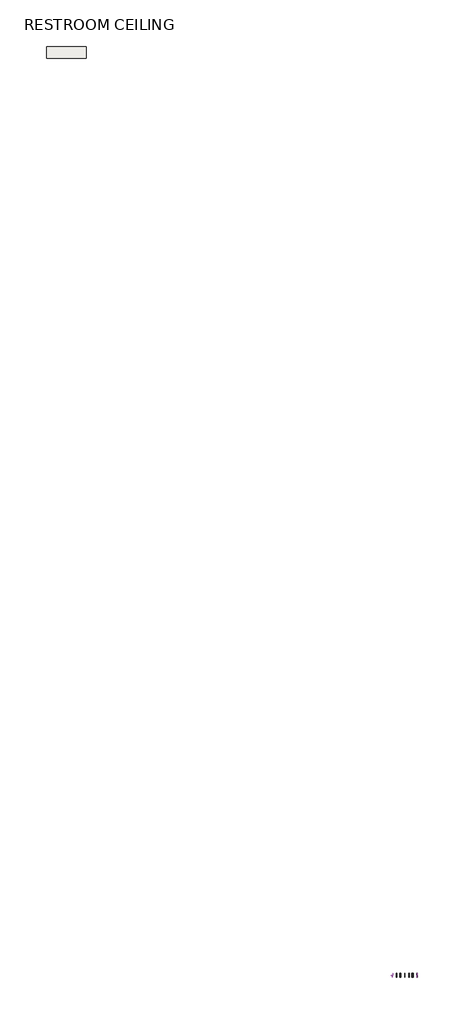
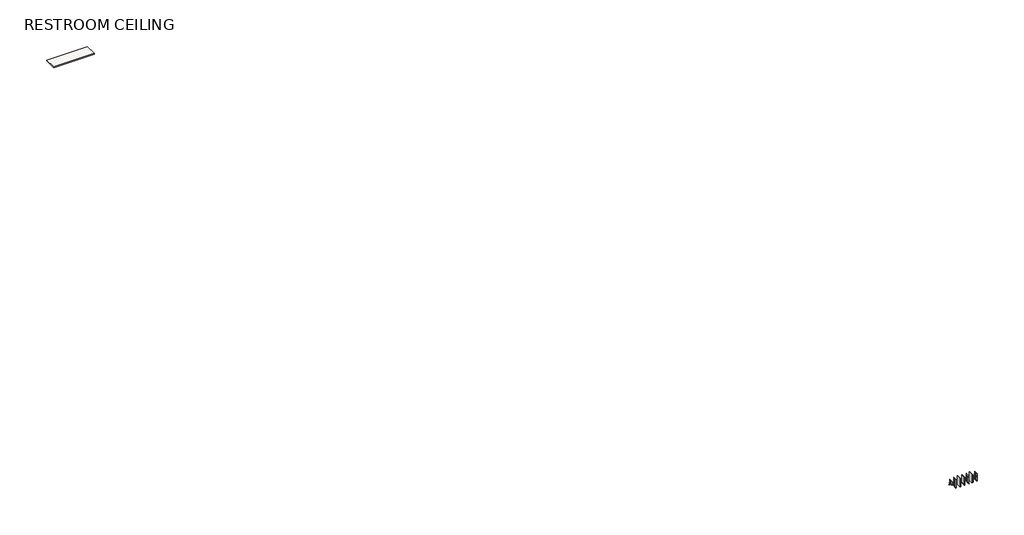
# One storey: 61 proxies, 1 slab.
"""IFC4 building model written with IfcOpenShell, lengths in millimetres."""

import ifcopenshell
import ifcopenshell.guid

model = None  # the IFC model being written
_history = None  # IfcOwnerHistory: only IFC2X3 demands one
_inside = {}  # id of a spatial element -> (the spatial element, [elements in it])
_under = {}  # id of a project, library or spatial element -> (it, [spatial elements below it])
_declared = {}  # id of a project -> (the project, [libraries it declares])
_typed = {}  # id of a type object -> (the type object, [elements of that type])
_made_of = {}  # id of a material, layer set ... -> (it, [elements and type objects made of it])


def new_model(schema):
    """Start an empty IFC model of exactly this schema.

    Asked for "IFC4X3", IfcOpenShell would pick the latest addendum, in which some entities
    have other attributes; the version numbers below select the first issue.
    IFC2X3 requires an IfcOwnerHistory on every rooted entity: one is made here for all.
    """
    global model, _history
    if schema == "IFC4X3":
        model = ifcopenshell.file(schema_version=(4, 3, 0, 0))
    else:
        model = ifcopenshell.file(schema=schema)
    _inside.clear()
    _under.clear()
    _declared.clear()
    _typed.clear()
    _made_of.clear()
    _history = None
    if model.schema == "IFC2X3":
        org = make("IfcOrganization", Name="unknown")
        user = make(
            "IfcPersonAndOrganization",
            ThePerson=make("IfcPerson", FamilyName="unknown"),
            TheOrganization=org,
        )
        app = make(
            "IfcApplication",
            ApplicationDeveloper=org,
            Version="unknown",
            ApplicationFullName="unknown",
            ApplicationIdentifier="unknown",
        )
        _history = make(
            "IfcOwnerHistory",
            OwningUser=user,
            OwningApplication=app,
            ChangeAction="ADDED",
            CreationDate=0,
        )
    return model


def make(cls, **values):
    """One entity of the class cls with the attributes given. An attribute that is None is left unset."""
    return model.create_entity(
        cls, **{name: value for name, value in values.items() if value is not None}
    )


def rooted(cls, **values):
    """An entity with a GlobalId (a new one), such as an element, a storey or a relation."""
    return make(cls, GlobalId=ifcopenshell.guid.new(), OwnerHistory=_history, **values)


def si_unit(unit_type, name, prefix=None):
    """IfcSIUnit, for example si_unit("LENGTHUNIT", "METRE", prefix="MILLI")."""
    return make("IfcSIUnit", UnitType=unit_type, Prefix=prefix, Name=name)


def assignment(units):
    """IfcUnitAssignment: the units of a project."""
    return None if units is None else make("IfcUnitAssignment", Units=units)


def point(xyz):
    """IfcCartesianPoint."""
    return None if xyz is None else make("IfcCartesianPoint", Coordinates=xyz)


def direction(xyz):
    """IfcDirection."""
    return None if xyz is None else make("IfcDirection", DirectionRatios=xyz)


def frame(location, z_axis=None, x_axis=None):
    """IfcAxis2Placement3D, a coordinate frame: its origin and axes. An axis left out is left unset."""
    return make(
        "IfcAxis2Placement3D",
        Location=point(location),
        Axis=direction(z_axis),
        RefDirection=direction(x_axis),
    )


def frame_2d(location, x_axis=None):
    """IfcAxis2Placement2D, a coordinate frame in the plane: its origin and x axis."""
    return make(
        "IfcAxis2Placement2D", Location=point(location), RefDirection=direction(x_axis)
    )


def origin():
    """The frame at (0, 0, 0) with its axes left unset."""
    return frame((0.0, 0.0, 0.0))


def place(relative_to, where):
    """IfcLocalPlacement: puts the frame where relative to a parent placement (None: the world)."""
    return make(
        "IfcLocalPlacement", PlacementRelTo=relative_to, RelativePlacement=where
    )


def context(
    kind, dimensions, precision=None, world=None, true_north=None, identifier=None
):
    """IfcGeometricRepresentationContext, for example the 3D "Model" context."""
    return make(
        "IfcGeometricRepresentationContext",
        ContextIdentifier=identifier,
        ContextType=kind,
        CoordinateSpaceDimension=dimensions,
        Precision=precision,
        WorldCoordinateSystem=world,
        TrueNorth=true_north,
    )


def project(units=None, contexts=None):
    """IfcProject with its units and contexts."""
    return rooted(
        "IfcProject",
        Name="project",
        RepresentationContexts=contexts,
        UnitsInContext=assignment(units),
    )


def spatial(cls, under=None, at=None, **own):
    """A site, building, storey or space (cls), placed at a placement, below another one or the project."""
    s = rooted(cls, ObjectPlacement=at, **own)
    if under is not None:
        _under.setdefault(under.id(), (under, []))[1].append(s)
    return s


def polyline(points):
    """IfcPolyline through the points."""
    return make("IfcPolyline", Points=[point(p) for p in points])


def circle_curve(where, radius):
    """IfcCircle in the frame where."""
    return make("IfcCircle", Position=where, Radius=radius)


def trimmed(basis, trim1, trim2, sense, master):
    """IfcTrimmedCurve: the piece of a basis curve between two trims."""
    return make(
        "IfcTrimmedCurve",
        BasisCurve=basis,
        Trim1=trim1,
        Trim2=trim2,
        SenseAgreement=sense,
        MasterRepresentation=master,
    )


def segment(curve, same_sense, transition):
    """IfcCompositeCurveSegment."""
    return make(
        "IfcCompositeCurveSegment",
        Transition=transition,
        SameSense=same_sense,
        ParentCurve=curve,
    )


def composite_curve(segments, self_intersect=None):
    """IfcCompositeCurve: segments joined end to end."""
    return make("IfcCompositeCurve", Segments=segments, SelfIntersect=self_intersect)


def outline(outer, holes=None, kind="AREA"):
    """IfcArbitraryClosedProfileDef: a profile drawn as a closed curve; with holes, ...WithVoids."""
    if holes is None:
        return make("IfcArbitraryClosedProfileDef", ProfileType=kind, OuterCurve=outer)
    return make(
        "IfcArbitraryProfileDefWithVoids",
        ProfileType=kind,
        OuterCurve=outer,
        InnerCurves=holes,
    )


def extrude(swept, where, along, depth):
    """IfcExtrudedAreaSolid: the profile swept, set in the frame where, extruded along a direction by depth."""
    return make(
        "IfcExtrudedAreaSolid",
        SweptArea=swept,
        Position=where,
        ExtrudedDirection=direction(along),
        Depth=depth,
    )


def shape(context_of_items, identifier, shape_type, items):
    """IfcShapeRepresentation: the items that make up one representation, for example the "Body"."""
    return make(
        "IfcShapeRepresentation",
        ContextOfItems=context_of_items,
        RepresentationIdentifier=identifier,
        RepresentationType=shape_type,
        Items=items,
    )


def source(mapping_origin, context_of_items, identifier, shape_type, items):
    """IfcRepresentationMap: a shape defined once, which mapped items show again and again."""
    return make(
        "IfcRepresentationMap",
        MappingOrigin=mapping_origin,
        MappedRepresentation=shape(context_of_items, identifier, shape_type, items),
    )


def transform(
    local_origin,
    x_axis=None,
    y_axis=None,
    z_axis=None,
    scale=None,
    scale2=None,
    scale3=None,
    uniform=True,
):
    """IfcCartesianTransformationOperator3D, or its non-uniform kind. x_axis, y_axis, z_axis: its Axis1, 2, 3."""
    if uniform:
        return make(
            "IfcCartesianTransformationOperator3D",
            Axis1=direction(x_axis),
            Axis2=direction(y_axis),
            LocalOrigin=point(local_origin),
            Scale=scale,
            Axis3=direction(z_axis),
        )
    return make(
        "IfcCartesianTransformationOperator3DnonUniform",
        Axis1=direction(x_axis),
        Axis2=direction(y_axis),
        LocalOrigin=point(local_origin),
        Scale=scale,
        Axis3=direction(z_axis),
        Scale2=scale2,
        Scale3=scale3,
    )


def mapped(mapping_source, mapping_target):
    """IfcMappedItem: shows the shape of a source again, moved by a transform."""
    return make(
        "IfcMappedItem", MappingSource=mapping_source, MappingTarget=mapping_target
    )


def made_of(thing, what):
    """Note that an element or type object is made of a material, layer set ...; save() writes the relation."""
    if what is not None:
        _made_of.setdefault(what.id(), (what, []))[1].append(thing)
    return thing


def element(
    cls,
    number,
    at=None,
    inside=None,
    cuts=None,
    type_object=None,
    material=None,
    context=None,
    identifier="Body",
    shape_type=None,
    held_by="IfcProductDefinitionShape",
    body=None,
    shapes=None,
    **own,
):
    """One element of the class cls, such as IfcWall. Its Tag is "e" and its number.

    at: its placement. inside: the storey or other place that contains it. cuts: it is an
    opening in that element (IfcRelVoidsElement). A single representation is given by context,
    identifier, shape_type and body (its items); several are given by shapes. held_by: the class
    of the entity that holds the representations. save() writes the other relations.
    """
    e = rooted(cls, Tag="e%d" % number, ObjectPlacement=at, **own)
    if body is not None:
        shapes = [shape(context, identifier, shape_type, body)]
    if shapes is not None:
        e.Representation = make(held_by, Representations=shapes)
    if inside is not None:
        _inside.setdefault(inside.id(), (inside, []))[1].append(e)
    if cuts is not None:
        rooted(
            "IfcRelVoidsElement", RelatingBuildingElement=cuts, RelatedOpeningElement=e
        )
    if type_object is not None:
        _typed.setdefault(type_object.id(), (type_object, []))[1].append(e)
    return made_of(e, material)


def aggregate(whole, parts):
    """IfcRelAggregates: a whole, such as a stair, and the parts it consists of."""
    return rooted("IfcRelAggregates", RelatingObject=whole, RelatedObjects=parts)


def save(model, path):
    """Write the relations noted so far, then the file.

    IfcRelAggregates (storeys below a building ...), IfcRelContainedInSpatialStructure (elements
    in a storey), IfcRelDefinesByType, IfcRelAssociatesMaterial and IfcRelDeclares: one each for
    every whole, place, type object, material and project.
    """
    for whole, parts in _under.values():
        aggregate(whole, parts)
    for where, things in _inside.values():
        rooted(
            "IfcRelContainedInSpatialStructure",
            RelatedElements=things,
            RelatingStructure=where,
        )
    for kind, things in _typed.values():
        rooted("IfcRelDefinesByType", RelatedObjects=things, RelatingType=kind)
    for what, things in _made_of.values():
        rooted("IfcRelAssociatesMaterial", RelatedObjects=things, RelatingMaterial=what)
    for by, libraries in _declared.values():
        rooted("IfcRelDeclares", RelatingContext=by, RelatedDefinitions=libraries)
    model.write(path)


def generic_models_1_generic_models_1_05f3df34(model_context):
    return source(origin(), model_context, "Body", "SweptSolid", [
        extrude(outline(polyline([(49784.0, 0.0), (49695.1, 0.0), (49695.1, 1219.2), (49784.0, 1219.2), (49784.0, 0.0)])), frame((0.0, 0.0, 3048.0), z_axis=(0.0, 0.0, 1.0), x_axis=(1.0, 0.0, 0.0)), (0.0, 0.0, 1.0), 38.1),
    ])


def generic_models_100_generic_models_1_fed90478(model_context):
    return source(origin(), model_context, "Body", "SweptSolid", [
        extrude(outline(polyline([(52216.05, 1219.2), (52216.05, 0.0), (52139.85, 0.0), (52139.85, 1219.2), (52216.05, 1219.2)])), frame((0.0, 0.0, 3211.5125), z_axis=(0.0, 0.0, 1.0), x_axis=(1.0, 0.0, 0.0)), (0.0, 0.0, 1.0), 1155.7),
    ])


def generic_models_101_generic_models_65_cc6b61b5(model_context):
    return source(origin(), model_context, "Body", "SweptSolid", [
        extrude(outline(polyline([(52222.4, 592.1375), (52133.5, 592.1375), (52133.5, 630.2375), (52222.4, 630.2375), (52222.4, 592.1375)])), frame((0.0, 0.0, 3203.178125), z_axis=(0.0, 0.0, 1.0), x_axis=(1.0, 0.0, 0.0)), (0.0, 0.0, 1.0), 1943.1),
    ])


def generic_models_102_generic_models_1_8a2dd616(model_context):
    return source(origin(), model_context, "Body", "SweptSolid", [
        extrude(outline(composite_curve([segment(polyline([(4498.578125, 52222.4), (4510.823229, 52207.8068534), (4508.6950617, 52206.021109), (4497.282664, 52219.621875), (4414.3677682, 52219.621875)]), True, "CONTINUOUS"), segment(trimmed(circle_curve(frame_2d((4414.4412941, 52217.6381931)), 1.9850441), [point((4414.3677682, 52219.621875))], [point((4412.45625, 52217.6381931))], True, "CARTESIAN"), True, "CONTINUOUS"), segment(polyline([(4412.45625, 52217.6381931), (4412.45625, 52023.9610661)]), True, "CONTINUOUS"), segment(trimmed(circle_curve(frame_2d((4414.4419899, 52023.9610661)), 1.9857399), [point((4412.45625, 52023.9610661))], [point((4414.3365981, 52021.978125))], True, "CARTESIAN"), True, "CONTINUOUS"), segment(polyline([(4414.3365981, 52021.978125), (4497.282664, 52021.978125), (4508.718285, 52035.6065673), (4510.8464522, 52033.820823), (4498.578125, 52019.2), (4414.440625, 52019.2)]), True, "CONTINUOUS"), segment(trimmed(circle_curve(frame_2d((4414.440625, 52023.9625)), 4.7625), [point((4414.440625, 52019.2))], [point((4409.678125, 52023.9625))], False, "CARTESIAN"), True, "CONTINUOUS"), segment(polyline([(4409.678125, 52023.9625), (4409.678125, 52217.6375)]), True, "CONTINUOUS"), segment(trimmed(circle_curve(frame_2d((4414.440625, 52217.6375)), 4.7625), [point((4409.678125, 52217.6375))], [point((4414.440625, 52222.4))], False, "CARTESIAN"), True, "CONTINUOUS"), segment(polyline([(4414.440625, 52222.4), (4498.578125, 52222.4)]), True, "CONTINUOUS")], self_intersect=False)), frame((0.0, 0.0, 0.0), z_axis=(0.0, 1.0, 0.0), x_axis=(0.0, 0.0, 1.0)), (0.0, 0.0, 1.0), 1219.2),
    ])


def generic_models_103_generic_models_1_250a6a11(model_context):
    return source(origin(), model_context, "Body", "SweptSolid", [
        extrude(outline(polyline([(49784.0, 0.0), (49695.1, 0.0), (49695.1, 1219.2), (49784.0, 1219.2), (49784.0, 0.0)])), frame((0.0, 0.0, 5264.15), z_axis=(0.0, 0.0, 1.0), x_axis=(1.0, 0.0, 0.0)), (0.0, 0.0, 1.0), 38.1),
    ])


def generic_models_104_generic_models_1_af33e5d9(model_context):
    return source(origin(), model_context, "Body", "SweptSolid", [
        extrude(outline(polyline([(52206.021109, 0.0), (52117.121109, 0.0), (52117.121109, 1219.2), (52206.021109, 1219.2), (52206.021109, 0.0)])), frame((0.0, 0.0, 4412.45625), z_axis=(0.0, 0.0, 1.0), x_axis=(1.0, 0.0, 0.0)), (0.0, 0.0, 1.0), 38.1),
    ])


def generic_models_108_generic_models_1_496acf5e(model_context):
    return source(origin(), model_context, "Body", "SweptSolid", [
        extrude(outline(polyline([(52216.05, 1219.2), (52216.05, 0.0), (52139.85, 0.0), (52139.85, 1219.2), (52216.05, 1219.2)])), frame((0.0, 0.0, 4570.4125), z_axis=(0.0, 0.0, 1.0), x_axis=(1.0, 0.0, 0.0)), (0.0, 0.0, 1.0), 565.15),
    ])


def generic_models_157_generic_models_1_b3b9a6c0(model_context):
    return source(origin(), model_context, "Body", "SweptSolid", [
        extrude(outline(polyline([(47363.0625, 1219.2), (47363.0625, 0.0), (47347.1875, 0.0), (47347.1875, 1219.2), (47363.0625, 1219.2)])), frame((0.0, 0.0, 4267.2), z_axis=(0.0, 0.0, 1.0), x_axis=(1.0, 0.0, 0.0)), (0.0, 0.0, 1.0), 1123.95),
    ])


def generic_models_2_generic_models_1_35b0c06a(model_context):
    return source(origin(), model_context, "Body", "SweptSolid", [
        extrude(outline(polyline([(49799.875, 1219.2), (49799.875, 0.0), (49784.0, 0.0), (49784.0, 1219.2), (49799.875, 1219.2)])), frame((0.0, 0.0, 3054.35), z_axis=(0.0, 0.0, 1.0), x_axis=(1.0, 0.0, 0.0)), (0.0, 0.0, 1.0), 2438.4),
    ])


def generic_models_216_generic_models_1_bf22bbd9(model_context):
    return source(origin(), model_context, "Body", "SweptSolid", [
        extrude(outline(polyline([(48582.2625, 1219.2), (48582.2625, 0.0), (48566.3875, 0.0), (48566.3875, 1219.2), (48582.2625, 1219.2)])), frame((0.0, 0.0, 3054.35), z_axis=(0.0, 0.0, 1.0), x_axis=(1.0, 0.0, 0.0)), (0.0, 0.0, 1.0), 2336.8),
    ])


def generic_models_17_generic_models_1_5a74d62d(model_context):
    return source(origin(), model_context, "Body", "SweptSolid", [
        extrude(outline(composite_curve([segment(trimmed(circle_curve(frame_2d((3.175, 49802.7897405)), 4.3100275), [point((0.0, 49799.875))], [point((6.35, 49799.875))], True, "CARTESIAN"), True, "CONTINUOUS"), segment(polyline([(6.35, 49799.875), (6.35, 49790.35)]), True, "CONTINUOUS"), segment(trimmed(circle_curve(frame_2d((3.175, 49793.2647405)), 4.3100275), [point((6.35, 49790.35))], [point((0.0, 49790.35))], False, "CARTESIAN"), True, "CONTINUOUS"), segment(polyline([(0.0, 49790.35), (0.0, 49799.875)]), True, "CONTINUOUS")], self_intersect=False)), frame((0.0, 0.0, 0.0), z_axis=(0.0, 1.0, 0.0), x_axis=(0.0, 0.0, 1.0)), (0.0, 0.0, 1.0), 1219.2),
    ])


def generic_models_186_generic_models_1_ef70466a(model_context):
    return source(origin(), model_context, "Body", "SweptSolid", [
        extrude(outline(composite_curve([segment(polyline([(101.6, 49799.875), (15.4496307, 49799.875)]), True, "CONTINUOUS"), segment(trimmed(circle_curve(frame_2d((15.4496307, 49817.7146968)), 17.8396968), [point((15.4496307, 49799.875))], [point((0.0, 49808.7948484))], False, "CARTESIAN"), True, "CONTINUOUS"), segment(polyline([(0.0, 49808.7948484), (2.7496307, 49810.3823484)]), True, "CONTINUOUS"), segment(trimmed(circle_curve(frame_2d((15.4496307, 49817.7146968)), 14.6646968), [point((2.7496307, 49810.3823484))], [point((15.4496307, 49803.05))], True, "CARTESIAN"), True, "CONTINUOUS"), segment(polyline([(15.4496307, 49803.05), (99.5131982, 49803.05)]), True, "CONTINUOUS"), segment(trimmed(circle_curve(frame_2d((99.5131982, 49800.9631982)), 2.0868018), [point((99.5131982, 49803.05))], [point((101.6, 49800.9631982))], False, "CARTESIAN"), True, "CONTINUOUS"), segment(polyline([(101.6, 49800.9631982), (101.6, 49799.875)]), True, "CONTINUOUS")], self_intersect=False)), frame((0.0, 0.0, 0.0), z_axis=(0.0, 1.0, 0.0), x_axis=(0.0, 0.0, 1.0)), (0.0, 0.0, 1.0), 1219.2),
    ])


def generic_models_227_generic_models_46_e0d4e21f(model_context):
    return source(origin(), model_context, "Body", "SweptSolid", [
        extrude(outline(polyline([(48566.0211605, 0.0), (48565.2274105, 0.0), (48565.2274105, 1219.2), (48566.0211605, 1219.2), (48566.0211605, 0.0)])), frame((0.0, 0.0, 3049.1358009), z_axis=(0.0, 0.0, 1.0), x_axis=(1.0, 0.0, 0.0)), (0.0, 0.0, 1.0), 2456.7781344),
    ])


def generic_models_228_generic_models_1_053e8907(model_context):
    return source(origin(), model_context, "Body", "SweptSolid", [
        extrude(outline(composite_curve([segment(polyline([(592.1375, 4235.45), (592.1375, 4267.2)]), True, "CONTINUOUS"), segment(trimmed(circle_curve(frame_2d((592.1375, 4264.025)), 3.175), [point((592.1375, 4267.2))], [point((595.3125, 4264.025))], False, "CARTESIAN"), True, "CONTINUOUS"), segment(polyline([(595.3125, 4264.025), (595.3125, 4240.2125)]), True, "CONTINUOUS"), segment(trimmed(circle_curve(frame_2d((596.9, 4240.2125)), 1.5875), [point((595.3125, 4240.2125))], [point((596.9, 4238.625))], True, "CARTESIAN"), True, "CONTINUOUS"), segment(polyline([(596.9, 4238.625), (620.7125, 4238.625)]), True, "CONTINUOUS"), segment(trimmed(circle_curve(frame_2d((620.7125, 4235.45)), 3.175), [point((620.7125, 4238.625))], [point((623.8875, 4235.45))], False, "CARTESIAN"), True, "CONTINUOUS"), segment(polyline([(623.8875, 4235.45), (592.1375, 4235.45)]), True, "CONTINUOUS")], self_intersect=False)), frame((46753.4625, 0.0, 0.0), z_axis=(1.0, 0.0, 0.0), x_axis=(0.0, 1.0, 0.0)), (0.0, 0.0, 1.0), 609.6),
    ])


def generic_models_232_generic_models_1_b4b06e59(model_context):
    return source(origin(), model_context, "Body", "SweptSolid", [
        extrude(outline(polyline([(49777.65, 1219.2), (49777.65, 0.0), (49701.45, 0.0), (49701.45, 1219.2), (49777.65, 1219.2)])), frame((0.0, 0.0, 3090.8625), z_axis=(0.0, 0.0, 1.0), x_axis=(1.0, 0.0, 0.0)), (0.0, 0.0, 1.0), 2368.55),
    ])


def generic_models_234_generic_models_65_886ed74c(model_context):
    return source(origin(), model_context, "Body", "SweptSolid", [
        extrude(outline(polyline([(49784.0, 592.1375), (49695.1, 592.1375), (49695.1, 630.2375), (49784.0, 630.2375), (49784.0, 592.1375)])), frame((0.0, 0.0, 3086.1), z_axis=(0.0, 0.0, 1.0), x_axis=(1.0, 0.0, 0.0)), (0.0, 0.0, 1.0), 2381.25),
    ])


def generic_models_241_generic_models_1_d4f8735c(model_context):
    return source(origin(), model_context, "Body", "SweptSolid", [
        extrude(outline(polyline([(48469.55, 1219.2), (48469.55, 0.0), (48317.15, 0.0), (48317.15, 1219.2), (48469.55, 1219.2)])), frame((0.0, 0.0, 3048.0), z_axis=(0.0, 0.0, 1.0), x_axis=(1.0, 0.0, 0.0)), (0.0, 0.0, 1.0), 2633.9569015),
    ])


def generic_models_246_generic_models_1_33f707d8(model_context):
    return source(origin(), model_context, "Body", "SweptSolid", [
        extrude(outline(composite_curve([segment(polyline([(4267.2, 47363.0625), (4267.2, 47331.3125)]), True, "CONTINUOUS"), segment(trimmed(circle_curve(frame_2d((4267.2, 47334.4875)), 3.175), [point((4267.2, 47331.3125))], [point((4264.025, 47334.4875))], False, "CARTESIAN"), True, "CONTINUOUS"), segment(polyline([(4264.025, 47334.4875), (4264.025, 47358.3)]), True, "CONTINUOUS"), segment(trimmed(circle_curve(frame_2d((4262.4375, 47358.3)), 1.5875), [point((4264.025, 47358.3))], [point((4262.4375, 47359.8875))], True, "CARTESIAN"), True, "CONTINUOUS"), segment(polyline([(4262.4375, 47359.8875), (4238.625, 47359.8875)]), True, "CONTINUOUS"), segment(trimmed(circle_curve(frame_2d((4238.625, 47363.0625)), 3.175), [point((4238.625, 47359.8875))], [point((4235.45, 47363.0625))], False, "CARTESIAN"), True, "CONTINUOUS"), segment(polyline([(4235.45, 47363.0625), (4267.2, 47363.0625)]), True, "CONTINUOUS")], self_intersect=False)), frame((0.0, 0.0, 0.0), z_axis=(0.0, 1.0, 0.0), x_axis=(0.0, 0.0, 1.0)), (0.0, 0.0, 1.0), 1219.2),
    ])


def generic_models_248_generic_models_65_f6c484d7(model_context):
    return source(origin(), model_context, "Body", "SweptSolid", [
        extrude(outline(polyline([(47345.6, 592.1375), (47256.7, 592.1375), (47256.7, 630.2375), (47345.6, 630.2375), (47345.6, 592.1375)])), frame((0.0, 0.0, 4305.3), z_axis=(0.0, 0.0, 1.0), x_axis=(1.0, 0.0, 0.0)), (0.0, 0.0, 1.0), 1162.05),
    ])


def generic_models_195_generic_models_1_9bd07d6e(model_context):
    return source(origin(), model_context, "Body", "SweptSolid", [
        extrude(outline(composite_curve([segment(polyline([(0.0, 49676.05), (0.0, 49685.575)]), True, "CONTINUOUS"), segment(trimmed(circle_curve(frame_2d((3.175, 49682.6602595)), 4.3100275), [point((0.0, 49685.575))], [point((6.35, 49685.575))], False, "CARTESIAN"), True, "CONTINUOUS"), segment(polyline([(6.35, 49685.575), (6.35, 49676.05)]), True, "CONTINUOUS"), segment(trimmed(circle_curve(frame_2d((3.175, 49673.1352595)), 4.3100275), [point((6.35, 49676.05))], [point((0.0, 49676.05))], True, "CARTESIAN"), True, "CONTINUOUS")], self_intersect=False)), frame((0.0, 0.0, 0.0), z_axis=(0.0, 1.0, 0.0), x_axis=(0.0, 0.0, 1.0)), (0.0, 0.0, 1.0), 1219.2),
    ])


def generic_models_196_generic_models_1_c5b7b2a8(model_context):
    return source(origin(), model_context, "Body", "SweptSolid", [
        extrude(outline(composite_curve([segment(polyline([(101.6, 49676.05), (101.6, 49674.9618018)]), True, "CONTINUOUS"), segment(trimmed(circle_curve(frame_2d((99.5131982, 49674.9618018)), 2.0868018), [point((101.6, 49674.9618018))], [point((99.5131982, 49672.875))], False, "CARTESIAN"), True, "CONTINUOUS"), segment(polyline([(99.5131982, 49672.875), (15.4496307, 49672.875)]), True, "CONTINUOUS"), segment(trimmed(circle_curve(frame_2d((15.4496307, 49658.2103032)), 14.6646968), [point((15.4496307, 49672.875))], [point((2.7496307, 49665.5426516))], True, "CARTESIAN"), True, "CONTINUOUS"), segment(polyline([(2.7496307, 49665.5426516), (0.0, 49667.1301516)]), True, "CONTINUOUS"), segment(trimmed(circle_curve(frame_2d((15.4496307, 49658.2103032)), 17.8396968), [point((0.0, 49667.1301516))], [point((15.4496307, 49676.05))], False, "CARTESIAN"), True, "CONTINUOUS"), segment(polyline([(15.4496307, 49676.05), (101.6, 49676.05)]), True, "CONTINUOUS")], self_intersect=False)), frame((0.0, 0.0, 0.0), z_axis=(0.0, 1.0, 0.0), x_axis=(0.0, 0.0, 1.0)), (0.0, 0.0, 1.0), 1219.2),
    ])


def generic_models_44_generic_models_1_ce885a63(model_context):
    return source(origin(), model_context, "Body", "SweptSolid", [
        extrude(outline(polyline([(51019.075, 1219.2), (51019.075, 0.0), (51003.2, 0.0), (51003.2, 1219.2), (51019.075, 1219.2)])), frame((0.0, 0.0, 3054.35), z_axis=(0.0, 0.0, 1.0), x_axis=(1.0, 0.0, 0.0)), (0.0, 0.0, 1.0), 2168.128125),
    ])


def generic_models_55_generic_models_1_42571d6e(model_context):
    return source(origin(), model_context, "Body", "SweptSolid", [
        extrude(outline(polyline([(52238.275, 1219.2), (52238.275, 0.0), (52222.4, 0.0), (52222.4, 1219.2), (52238.275, 1219.2)])), frame((0.0, 0.0, 3054.35), z_axis=(0.0, 0.0, 1.0), x_axis=(1.0, 0.0, 0.0)), (0.0, 0.0, 1.0), 2168.128125),
    ])


def generic_models_63_generic_models_1_f1177d32(model_context):
    return source(origin(), model_context, "Body", "SweptSolid", [
        extrude(outline(polyline([(50996.85, 1219.2), (50996.85, 0.0), (50920.65, 0.0), (50920.65, 1219.2), (50996.85, 1219.2)])), frame((0.0, 0.0, 3090.8625), z_axis=(0.0, 0.0, 1.0), x_axis=(1.0, 0.0, 0.0)), (0.0, 0.0, 1.0), 2044.7),
    ])


def generic_models_65_generic_models_65_eaa428f0(model_context):
    return source(origin(), model_context, "Body", "SweptSolid", [
        extrude(outline(polyline([(51003.2, 592.1375), (50914.3, 592.1375), (50914.3, 630.2375), (51003.2, 630.2375), (51003.2, 592.1375)])), frame((0.0, 0.0, 3086.1), z_axis=(0.0, 0.0, 1.0), x_axis=(1.0, 0.0, 0.0)), (0.0, 0.0, 1.0), 2060.178125),
    ])


def generic_models_69_generic_models_1_75d49a3d(model_context):
    return source(origin(), model_context, "Body", "SweptSolid", [
        extrude(outline(polyline([(50914.3, 1219.2), (50914.3, 0.0), (50898.425, 0.0), (50898.425, 1219.2), (50914.3, 1219.2)])), frame((0.0, 0.0, 3054.35), z_axis=(0.0, 0.0, 1.0), x_axis=(1.0, 0.0, 0.0)), (0.0, 0.0, 1.0), 2472.928125),
    ])


def generic_models_76_generic_models_1_e0c76cb0(model_context):
    return source(origin(), model_context, "Body", "SweptSolid", [
        extrude(outline(polyline([(51930.3, 1219.2), (51930.3, 0.0), (51777.9, 0.0), (51777.9, 1219.2), (51930.3, 1219.2)])), frame((0.0, 0.0, 3048.0), z_axis=(0.0, 0.0, 1.0), x_axis=(1.0, 0.0, 0.0)), (0.0, 0.0, 1.0), 2633.9569015),
    ])


def generic_models_85_generic_models_65_bcc3fffd(model_context):
    return source(origin(), model_context, "Body", "SweptSolid", [
        extrude(outline(polyline([(52222.4, 592.1375), (52133.5, 592.1375), (52133.5, 630.2375), (52222.4, 630.2375), (52222.4, 592.1375)])), frame((0.0, 0.0, 3086.1), z_axis=(0.0, 0.0, 1.0), x_axis=(1.0, 0.0, 0.0)), (0.0, 0.0, 1.0), 2098.278125),
    ])


model = new_model("IFC4")

# Units and contexts
model_context = context("Model", 3, world=origin())
ifc_project = project(units=[si_unit("LENGTHUNIT", "METRE", prefix="MILLI")], contexts=[model_context])

# Site, building, storey
site = spatial("IfcSite", under=ifc_project)
building = spatial("IfcBuilding", under=site)
storey = spatial("IfcBuildingStorey", under=building, Name="RESTROOM CEILING", Elevation=3019.425)

# Proxies
placement = place(None, origin())
generic_models_1_generic_models_1_shape = generic_models_1_generic_models_1_05f3df34(model_context)
element("IfcBuildingElementProxy", 1, Name="Generic Models 1 : Generic Models 1", ObjectType="Generic Models 1 : Generic Models 1", at=placement, inside=storey, context=model_context, shape_type="MappedRepresentation", body=[
    mapped(generic_models_1_generic_models_1_shape, transform((0.0, 0.0, 0.0), x_axis=(1.0, 0.0, 0.0), y_axis=(0.0, 1.0, 0.0), z_axis=(0.0, 0.0, 1.0))),
])
generic_models_100_generic_models_1_shape = generic_models_100_generic_models_1_fed90478(model_context)
element("IfcBuildingElementProxy", 2, Name="Generic Models 100 : Generic Models 1", ObjectType="Generic Models 100 : Generic Models 1", at=placement, inside=storey, context=model_context, shape_type="MappedRepresentation", body=[
    mapped(generic_models_100_generic_models_1_shape, transform((1219.2, 0.0, 0.0), x_axis=(1.0, 0.0, 0.0), y_axis=(0.0, 1.0, 0.0), z_axis=(0.0, 0.0, 1.0))),
])
generic_models_101_generic_models_65_shape = generic_models_101_generic_models_65_cc6b61b5(model_context)
element("IfcBuildingElementProxy", 3, Name="Generic Models 101 : Generic Models 65", ObjectType="Generic Models 101 : Generic Models 65", at=placement, inside=storey, context=model_context, shape_type="MappedRepresentation", body=[
    mapped(generic_models_101_generic_models_65_shape, transform((1219.2, 0.0, 0.0), x_axis=(1.0, 0.0, 0.0), y_axis=(0.0, 1.0, 0.0), z_axis=(0.0, 0.0, 1.0))),
])
generic_models_102_generic_models_1_shape = generic_models_102_generic_models_1_8a2dd616(model_context)
element("IfcBuildingElementProxy", 4, Name="Generic Models 102 : Generic Models 1", ObjectType="Generic Models 102 : Generic Models 1", at=placement, inside=storey, context=model_context, shape_type="MappedRepresentation", body=[
    mapped(generic_models_102_generic_models_1_shape, transform((1219.2, 0.0, 0.0), x_axis=(1.0, 0.0, 0.0), y_axis=(0.0, 1.0, 0.0), z_axis=(0.0, 0.0, 1.0))),
])
generic_models_103_generic_models_1_shape = generic_models_103_generic_models_1_250a6a11(model_context)
element("IfcBuildingElementProxy", 5, Name="Generic Models 103 : Generic Models 1", ObjectType="Generic Models 103 : Generic Models 1", at=placement, inside=storey, context=model_context, shape_type="MappedRepresentation", body=[
    mapped(generic_models_103_generic_models_1_shape, transform((3657.6, 0.0, -892.571875), x_axis=(1.0, 0.0, 0.0), y_axis=(0.0, 1.0, 0.0), z_axis=(0.0, 0.0, 1.0))),
])
generic_models_104_generic_models_1_shape = generic_models_104_generic_models_1_af33e5d9(model_context)
element("IfcBuildingElementProxy", 6, Name="Generic Models 104 : Generic Models 1", ObjectType="Generic Models 104 : Generic Models 1", at=placement, inside=storey, context=model_context, shape_type="MappedRepresentation", body=[
    mapped(generic_models_104_generic_models_1_shape, transform((1219.2, 0.0, 0.0), x_axis=(1.0, 0.0, 0.0), y_axis=(0.0, 1.0, 0.0), z_axis=(0.0, 0.0, 1.0))),
])
element("IfcBuildingElementProxy", 7, Name="Generic Models 105 : Generic Models 1", ObjectType="Generic Models 105 : Generic Models 1", at=placement, inside=storey, context=model_context, shape_type="MappedRepresentation", body=[
    mapped(generic_models_103_generic_models_1_shape, transform((3641.221109, 0.0, -813.59375), x_axis=(1.0, 0.0, 0.0), y_axis=(0.0, 1.0, 0.0), z_axis=(0.0, 0.0, 1.0))),
])
element("IfcBuildingElementProxy", 8, Name="Generic Models 106 : Generic Models 1", ObjectType="Generic Models 106 : Generic Models 1", at=placement, inside=storey, context=model_context, shape_type="MappedRepresentation", body=[
    mapped(generic_models_103_generic_models_1_shape, transform((3641.221109, 0.0, -775.49375), x_axis=(1.0, 0.0, 0.0), y_axis=(0.0, 1.0, 0.0), z_axis=(0.0, 0.0, 1.0))),
])
element("IfcBuildingElementProxy", 9, Name="Generic Models 107 : Generic Models 1", ObjectType="Generic Models 107 : Generic Models 1", at=placement, inside=storey, context=model_context, shape_type="MappedRepresentation", body=[
    mapped(generic_models_103_generic_models_1_shape, transform((3657.6, 0.0, -737.39375), x_axis=(1.0, 0.0, 0.0), y_axis=(0.0, 1.0, 0.0), z_axis=(0.0, 0.0, 1.0))),
])
generic_models_108_generic_models_1_shape = generic_models_108_generic_models_1_496acf5e(model_context)
element("IfcBuildingElementProxy", 10, Name="Generic Models 108 : Generic Models 1", ObjectType="Generic Models 108 : Generic Models 1", at=placement, inside=storey, context=model_context, shape_type="MappedRepresentation", body=[
    mapped(generic_models_108_generic_models_1_shape, transform((1219.2, 0.0, 0.0), x_axis=(1.0, 0.0, 0.0), y_axis=(0.0, 1.0, 0.0), z_axis=(0.0, 0.0, 1.0))),
])
element("IfcBuildingElementProxy", 11, Name="Generic Models 116 : Generic Models 1", ObjectType="Generic Models 116 : Generic Models 1", at=placement, inside=storey, context=model_context, shape_type="MappedRepresentation", body=[
    mapped(generic_models_102_generic_models_1_shape, transform((1219.2, 0.0, -1361.678125), x_axis=(1.0, 0.0, 0.0), y_axis=(0.0, 1.0, 0.0), z_axis=(0.0, 0.0, 1.0))),
])
element("IfcBuildingElementProxy", 12, Name="Generic Models 117 : Generic Models 1", ObjectType="Generic Models 117 : Generic Models 1", at=placement, inside=storey, context=model_context, shape_type="MappedRepresentation", body=[
    mapped(generic_models_104_generic_models_1_shape, transform((1219.2, 0.0, -1361.678125), x_axis=(1.0, 0.0, 0.0), y_axis=(0.0, 1.0, 0.0), z_axis=(0.0, 0.0, 1.0))),
])
element("IfcBuildingElementProxy", 13, Name="Generic Models 118 : Generic Models 1", ObjectType="Generic Models 118 : Generic Models 1", at=placement, inside=storey, context=model_context, shape_type="MappedRepresentation", body=[
    mapped(generic_models_103_generic_models_1_shape, transform((3641.221109, 0.0, -2175.271875), x_axis=(1.0, 0.0, 0.0), y_axis=(0.0, 1.0, 0.0), z_axis=(0.0, 0.0, 1.0))),
])
element("IfcBuildingElementProxy", 14, Name="Generic Models 119 : Generic Models 1", ObjectType="Generic Models 119 : Generic Models 1", at=placement, inside=storey, context=model_context, shape_type="MappedRepresentation", body=[
    mapped(generic_models_103_generic_models_1_shape, transform((3641.221109, 0.0, -2137.171875), x_axis=(1.0, 0.0, 0.0), y_axis=(0.0, 1.0, 0.0), z_axis=(0.0, 0.0, 1.0))),
])
element("IfcBuildingElementProxy", 15, Name="Generic Models 120 : Generic Models 1", ObjectType="Generic Models 120 : Generic Models 1", at=placement, inside=storey, context=model_context, shape_type="MappedRepresentation", body=[
    mapped(generic_models_103_generic_models_1_shape, transform((3657.6, 0.0, -2099.071875), x_axis=(1.0, 0.0, 0.0), y_axis=(0.0, 1.0, 0.0), z_axis=(0.0, 0.0, 1.0))),
])
element("IfcBuildingElementProxy", 16, Name="Generic Models 155 : Generic Models 1", ObjectType="Generic Models 155 : Generic Models 1", at=placement, inside=storey, context=model_context, shape_type="MappedRepresentation", body=[
    mapped(generic_models_1_generic_models_1_shape, transform((-3657.6, 0.0, 1219.2), x_axis=(1.0, 0.0, 0.0), y_axis=(0.0, 1.0, 0.0), z_axis=(0.0, 0.0, 1.0))),
])
generic_models_157_generic_models_1_shape = generic_models_157_generic_models_1_b3b9a6c0(model_context)
element("IfcBuildingElementProxy", 17, Name="Generic Models 157 : Generic Models 1", ObjectType="Generic Models 157 : Generic Models 1", at=placement, inside=storey, context=model_context, shape_type="MappedRepresentation", body=[
    mapped(generic_models_157_generic_models_1_shape, transform((-1219.2, 0.0, 0.0), x_axis=(1.0, 0.0, 0.0), y_axis=(0.0, 1.0, 0.0), z_axis=(0.0, 0.0, 1.0))),
])
generic_models_2_generic_models_1_shape = generic_models_2_generic_models_1_35b0c06a(model_context)
element("IfcBuildingElementProxy", 18, Name="Generic Models 2 : Generic Models 1", ObjectType="Generic Models 2 : Generic Models 1", at=placement, inside=storey, context=model_context, shape_type="MappedRepresentation", body=[
    mapped(generic_models_2_generic_models_1_shape, transform((0.0, 0.0, 0.0), x_axis=(1.0, 0.0, 0.0), y_axis=(0.0, 1.0, 0.0), z_axis=(0.0, 0.0, 1.0))),
])
element("IfcBuildingElementProxy", 19, Name="Generic Models 215 : Generic Models 1", ObjectType="Generic Models 215 : Generic Models 1", at=placement, inside=storey, context=model_context, shape_type="MappedRepresentation", body=[
    mapped(generic_models_1_generic_models_1_shape, transform((-1219.2, 0.0, 0.0), x_axis=(1.0, 0.0, 0.0), y_axis=(0.0, 1.0, 0.0), z_axis=(0.0, 0.0, 1.0))),
])
generic_models_216_generic_models_1_shape = generic_models_216_generic_models_1_bf22bbd9(model_context)
element("IfcBuildingElementProxy", 20, Name="Generic Models 216 : Generic Models 1", ObjectType="Generic Models 216 : Generic Models 1", at=placement, inside=storey, context=model_context, shape_type="MappedRepresentation", body=[
    mapped(generic_models_216_generic_models_1_shape, transform((0.0, 0.0, 0.0), x_axis=(1.0, 0.0, 0.0), y_axis=(0.0, 1.0, 0.0), z_axis=(0.0, 0.0, 1.0))),
])
generic_models_17_generic_models_1_shape = generic_models_17_generic_models_1_5a74d62d(model_context)
element("IfcBuildingElementProxy", 21, Name="Generic Models 217 : Generic Models 1", ObjectType="Generic Models 217 : Generic Models 1", at=placement, inside=storey, context=model_context, shape_type="MappedRepresentation", body=[
    mapped(generic_models_17_generic_models_1_shape, transform((-1217.6125, 0.0, 3048.0), x_axis=(1.0, 0.0, 0.0), y_axis=(0.0, 1.0, 0.0), z_axis=(0.0, 0.0, 1.0))),
])
generic_models_186_generic_models_1_shape = generic_models_186_generic_models_1_ef70466a(model_context)
element("IfcBuildingElementProxy", 22, Name="Generic Models 222 : Generic Models 1", ObjectType="Generic Models 222 : Generic Models 1", at=placement, inside=storey, context=model_context, shape_type="MappedRepresentation", body=[
    mapped(generic_models_186_generic_models_1_shape, transform((-1217.6125, 0.0, 3048.0), x_axis=(1.0, 0.0, 0.0), y_axis=(0.0, 1.0, 0.0), z_axis=(0.0, 0.0, 1.0))),
])
generic_models_227_generic_models_46_shape = generic_models_227_generic_models_46_e0d4e21f(model_context)
element("IfcBuildingElementProxy", 23, Name="Generic Models 227 : Generic Models 46", ObjectType="Generic Models 227 : Generic Models 46", at=placement, inside=storey, context=model_context, shape_type="MappedRepresentation", body=[
    mapped(generic_models_227_generic_models_46_shape, transform((0.0, 0.0, 0.0), x_axis=(1.0, 0.0, 0.0), y_axis=(0.0, 1.0, 0.0), z_axis=(0.0, 0.0, 1.0))),
])
generic_models_228_generic_models_1_shape = generic_models_228_generic_models_1_053e8907(model_context)
element("IfcBuildingElementProxy", 24, Name="Generic Models 228 : Generic Models 1", ObjectType="Generic Models 228 : Generic Models 1", at=placement, inside=storey, context=model_context, shape_type="MappedRepresentation", body=[
    mapped(generic_models_228_generic_models_1_shape, transform((-1219.2, 0.0, 0.0), x_axis=(1.0, 0.0, 0.0), y_axis=(0.0, 1.0, 0.0), z_axis=(0.0, 0.0, 1.0))),
])
element("IfcBuildingElementProxy", 25, Name="Generic Models 229 : Generic Models 1", ObjectType="Generic Models 229 : Generic Models 1", at=placement, inside=storey, context=model_context, shape_type="MappedRepresentation", body=[
    mapped(generic_models_1_generic_models_1_shape, transform((-2438.4, 0.0, 0.0), x_axis=(1.0, 0.0, 0.0), y_axis=(0.0, 1.0, 0.0), z_axis=(0.0, 0.0, 1.0))),
])
generic_models_232_generic_models_1_shape = generic_models_232_generic_models_1_b4b06e59(model_context)
element("IfcBuildingElementProxy", 26, Name="Generic Models 232 : Generic Models 1", ObjectType="Generic Models 232 : Generic Models 1", at=placement, inside=storey, context=model_context, shape_type="MappedRepresentation", body=[
    mapped(generic_models_232_generic_models_1_shape, transform((-1219.2, 0.0, 0.0), x_axis=(1.0, 0.0, 0.0), y_axis=(0.0, 1.0, 0.0), z_axis=(0.0, 0.0, 1.0))),
])
generic_models_234_generic_models_65_shape = generic_models_234_generic_models_65_886ed74c(model_context)
element("IfcBuildingElementProxy", 27, Name="Generic Models 234 : Generic Models 65", ObjectType="Generic Models 234 : Generic Models 65", at=placement, inside=storey, context=model_context, shape_type="MappedRepresentation", body=[
    mapped(generic_models_234_generic_models_65_shape, transform((-1219.2, 0.0, 0.0), x_axis=(1.0, 0.0, 0.0), y_axis=(0.0, 1.0, 0.0), z_axis=(0.0, 0.0, 1.0))),
])
generic_models_241_generic_models_1_shape = generic_models_241_generic_models_1_d4f8735c(model_context)
element("IfcBuildingElementProxy", 28, Name="Generic Models 241 : Generic Models 1", ObjectType="Generic Models 241 : Generic Models 1", at=placement, inside=storey, context=model_context, shape_type="MappedRepresentation", body=[
    mapped(generic_models_241_generic_models_1_shape, transform((0.0, 0.0, 0.0), x_axis=(1.0, 0.0, 0.0), y_axis=(0.0, 1.0, 0.0), z_axis=(0.0, 0.0, 1.0))),
])
element("IfcBuildingElementProxy", 29, Name="Generic Models 244 : Generic Models 1", ObjectType="Generic Models 244 : Generic Models 1", at=placement, inside=storey, context=model_context, shape_type="MappedRepresentation", body=[
    mapped(generic_models_216_generic_models_1_shape, transform((-1219.2, 0.0, 0.0), x_axis=(1.0, 0.0, 0.0), y_axis=(0.0, 1.0, 0.0), z_axis=(0.0, 0.0, 1.0))),
])
generic_models_246_generic_models_1_shape = generic_models_246_generic_models_1_33f707d8(model_context)
element("IfcBuildingElementProxy", 30, Name="Generic Models 246 : Generic Models 1", ObjectType="Generic Models 246 : Generic Models 1", at=placement, inside=storey, context=model_context, shape_type="MappedRepresentation", body=[
    mapped(generic_models_246_generic_models_1_shape, transform((-1219.2, 0.0, 0.0), x_axis=(1.0, 0.0, 0.0), y_axis=(0.0, 1.0, 0.0), z_axis=(0.0, 0.0, 1.0))),
])
generic_models_248_generic_models_65_shape = generic_models_248_generic_models_65_f6c484d7(model_context)
element("IfcBuildingElementProxy", 31, Name="Generic Models 248 : Generic Models 65", ObjectType="Generic Models 248 : Generic Models 65", at=placement, inside=storey, context=model_context, shape_type="MappedRepresentation", body=[
    mapped(generic_models_248_generic_models_65_shape, transform((-1219.2, 0.0, 0.0), x_axis=(1.0, 0.0, 0.0), y_axis=(0.0, 1.0, 0.0), z_axis=(0.0, 0.0, 1.0))),
])
element("IfcBuildingElementProxy", 32, Name="Generic Models 249 : Generic Models 1", ObjectType="Generic Models 249 : Generic Models 1", at=placement, inside=storey, context=model_context, shape_type="MappedRepresentation", body=[
    mapped(generic_models_17_generic_models_1_shape, transform((-2436.8125, 0.0, 3048.0), x_axis=(1.0, 0.0, 0.0), y_axis=(0.0, 1.0, 0.0), z_axis=(0.0, 0.0, 1.0))),
])
element("IfcBuildingElementProxy", 33, Name="Generic Models 253 : Generic Models 1", ObjectType="Generic Models 253 : Generic Models 1", at=placement, inside=storey, context=model_context, shape_type="MappedRepresentation", body=[
    mapped(generic_models_186_generic_models_1_shape, transform((-2436.8125, 0.0, 3048.0), x_axis=(1.0, 0.0, 0.0), y_axis=(0.0, 1.0, 0.0), z_axis=(0.0, 0.0, 1.0))),
])
element("IfcBuildingElementProxy", 34, Name="Generic Models 260 : Generic Models 1", ObjectType="Generic Models 260 : Generic Models 1", at=placement, inside=storey, context=model_context, shape_type="MappedRepresentation", body=[
    mapped(generic_models_232_generic_models_1_shape, transform((-2438.4, 0.0, 0.0), x_axis=(1.0, 0.0, 0.0), y_axis=(0.0, 1.0, 0.0), z_axis=(0.0, 0.0, 1.0))),
])
element("IfcBuildingElementProxy", 35, Name="Generic Models 262 : Generic Models 65", ObjectType="Generic Models 262 : Generic Models 65", at=placement, inside=storey, context=model_context, shape_type="MappedRepresentation", body=[
    mapped(generic_models_234_generic_models_65_shape, transform((-2438.4, 0.0, 0.0), x_axis=(1.0, 0.0, 0.0), y_axis=(0.0, 1.0, 0.0), z_axis=(0.0, 0.0, 1.0))),
])
element("IfcBuildingElementProxy", 36, Name="Generic Models 268 : Generic Models 46", ObjectType="Generic Models 268 : Generic Models 46", at=placement, inside=storey, context=model_context, shape_type="MappedRepresentation", body=[
    mapped(generic_models_227_generic_models_46_shape, transform((-1219.2, 0.0, 0.0), x_axis=(1.0, 0.0, 0.0), y_axis=(0.0, 1.0, 0.0), z_axis=(0.0, 0.0, 1.0))),
])
element("IfcBuildingElementProxy", 37, Name="Generic Models 3 : Generic Models 1", ObjectType="Generic Models 3 : Generic Models 1", at=placement, inside=storey, context=model_context, shape_type="MappedRepresentation", body=[
    mapped(generic_models_17_generic_models_1_shape, transform((0.0, 0.0, 3048.0), x_axis=(1.0, 0.0, 0.0), y_axis=(0.0, 1.0, 0.0), z_axis=(0.0, 0.0, 1.0))),
])
element("IfcBuildingElementProxy", 38, Name="Generic Models 40 : Generic Models 1", ObjectType="Generic Models 40 : Generic Models 1", at=placement, inside=storey, context=model_context, shape_type="MappedRepresentation", body=[
    mapped(generic_models_1_generic_models_1_shape, transform((1219.2, 0.0, 0.0), x_axis=(1.0, 0.0, 0.0), y_axis=(0.0, 1.0, 0.0), z_axis=(0.0, 0.0, 1.0))),
])
generic_models_195_generic_models_1_shape = generic_models_195_generic_models_1_9bd07d6e(model_context)
element("IfcBuildingElementProxy", 39, Name="Generic Models 41 : Generic Models 1", ObjectType="Generic Models 41 : Generic Models 1", at=placement, inside=storey, context=model_context, shape_type="MappedRepresentation", body=[
    mapped(generic_models_195_generic_models_1_shape, transform((3.175, 0.0, 3048.0), x_axis=(1.0, 0.0, 0.0), y_axis=(0.0, 1.0, 0.0), z_axis=(0.0, 0.0, 1.0))),
])
generic_models_196_generic_models_1_shape = generic_models_196_generic_models_1_c5b7b2a8(model_context)
element("IfcBuildingElementProxy", 40, Name="Generic Models 42 : Generic Models 1", ObjectType="Generic Models 42 : Generic Models 1", at=placement, inside=storey, context=model_context, shape_type="MappedRepresentation", body=[
    mapped(generic_models_196_generic_models_1_shape, transform((3.175, 0.0, 3048.0), x_axis=(1.0, 0.0, 0.0), y_axis=(0.0, 1.0, 0.0), z_axis=(0.0, 0.0, 1.0))),
])
generic_models_44_generic_models_1_shape = generic_models_44_generic_models_1_ce885a63(model_context)
element("IfcBuildingElementProxy", 41, Name="Generic Models 44 : Generic Models 1", ObjectType="Generic Models 44 : Generic Models 1", at=placement, inside=storey, context=model_context, shape_type="MappedRepresentation", body=[
    mapped(generic_models_44_generic_models_1_shape, transform((0.0, 0.0, 0.0), x_axis=(1.0, 0.0, 0.0), y_axis=(0.0, 1.0, 0.0), z_axis=(0.0, 0.0, 1.0))),
])
element("IfcBuildingElementProxy", 42, Name="Generic Models 45 : Generic Models 1", ObjectType="Generic Models 45 : Generic Models 1", at=placement, inside=storey, context=model_context, shape_type="MappedRepresentation", body=[
    mapped(generic_models_17_generic_models_1_shape, transform((1219.2, 0.0, 3048.0), x_axis=(1.0, 0.0, 0.0), y_axis=(0.0, 1.0, 0.0), z_axis=(0.0, 0.0, 1.0))),
])
element("IfcBuildingElementProxy", 43, Name="Generic Models 5 : Generic Models 1", ObjectType="Generic Models 5 : Generic Models 1", at=placement, inside=storey, context=model_context, shape_type="MappedRepresentation", body=[
    mapped(generic_models_186_generic_models_1_shape, transform((0.0, 0.0, 3048.0), x_axis=(1.0, 0.0, 0.0), y_axis=(0.0, 1.0, 0.0), z_axis=(0.0, 0.0, 1.0))),
])
element("IfcBuildingElementProxy", 44, Name="Generic Models 50 : Generic Models 1", ObjectType="Generic Models 50 : Generic Models 1", at=placement, inside=storey, context=model_context, shape_type="MappedRepresentation", body=[
    mapped(generic_models_186_generic_models_1_shape, transform((1219.2, 0.0, 3048.0), x_axis=(1.0, 0.0, 0.0), y_axis=(0.0, 1.0, 0.0), z_axis=(0.0, 0.0, 1.0))),
])
element("IfcBuildingElementProxy", 45, Name="Generic Models 52 : Generic Models 65", ObjectType="Generic Models 52 : Generic Models 65", at=placement, inside=storey, context=model_context, shape_type="MappedRepresentation", body=[
    mapped(generic_models_234_generic_models_65_shape, transform((0.0, 0.0, 0.0), x_axis=(1.0, 0.0, 0.0), y_axis=(0.0, 1.0, 0.0), z_axis=(0.0, 0.0, 1.0))),
])
generic_models_55_generic_models_1_shape = generic_models_55_generic_models_1_42571d6e(model_context)
element("IfcBuildingElementProxy", 46, Name="Generic Models 55 : Generic Models 1", ObjectType="Generic Models 55 : Generic Models 1", at=placement, inside=storey, context=model_context, shape_type="MappedRepresentation", body=[
    mapped(generic_models_55_generic_models_1_shape, transform((1219.2, 0.0, 0.0), x_axis=(1.0, 0.0, 0.0), y_axis=(0.0, 1.0, 0.0), z_axis=(0.0, 0.0, 1.0))),
])
element("IfcBuildingElementProxy", 47, Name="Generic Models 56 : Generic Models 1", ObjectType="Generic Models 56 : Generic Models 1", at=placement, inside=storey, context=model_context, shape_type="MappedRepresentation", body=[
    mapped(generic_models_1_generic_models_1_shape, transform((2438.4, 0.0, 0.0), x_axis=(1.0, 0.0, 0.0), y_axis=(0.0, 1.0, 0.0), z_axis=(0.0, 0.0, 1.0))),
])
element("IfcBuildingElementProxy", 48, Name="Generic Models 57 : Generic Models 1", ObjectType="Generic Models 57 : Generic Models 1", at=placement, inside=storey, context=model_context, shape_type="MappedRepresentation", body=[
    mapped(generic_models_195_generic_models_1_shape, transform((1222.375, 0.0, 3048.0), x_axis=(1.0, 0.0, 0.0), y_axis=(0.0, 1.0, 0.0), z_axis=(0.0, 0.0, 1.0))),
])
element("IfcBuildingElementProxy", 49, Name="Generic Models 58 : Generic Models 1", ObjectType="Generic Models 58 : Generic Models 1", at=placement, inside=storey, context=model_context, shape_type="MappedRepresentation", body=[
    mapped(generic_models_196_generic_models_1_shape, transform((1222.375, 0.0, 3048.0), x_axis=(1.0, 0.0, 0.0), y_axis=(0.0, 1.0, 0.0), z_axis=(0.0, 0.0, 1.0))),
])
element("IfcBuildingElementProxy", 50, Name="Generic Models 60 : Generic Models 1", ObjectType="Generic Models 60 : Generic Models 1", at=placement, inside=storey, context=model_context, shape_type="MappedRepresentation", body=[
    mapped(generic_models_44_generic_models_1_shape, transform((1219.2, 0.0, 0.0), x_axis=(1.0, 0.0, 0.0), y_axis=(0.0, 1.0, 0.0), z_axis=(0.0, 0.0, 1.0))),
])
generic_models_63_generic_models_1_shape = generic_models_63_generic_models_1_f1177d32(model_context)
element("IfcBuildingElementProxy", 51, Name="Generic Models 63 : Generic Models 1", ObjectType="Generic Models 63 : Generic Models 1", at=placement, inside=storey, context=model_context, shape_type="MappedRepresentation", body=[
    mapped(generic_models_63_generic_models_1_shape, transform((0.0, 0.0, 0.0), x_axis=(1.0, 0.0, 0.0), y_axis=(0.0, 1.0, 0.0), z_axis=(0.0, 0.0, 1.0))),
])
generic_models_65_generic_models_65_shape = generic_models_65_generic_models_65_eaa428f0(model_context)
element("IfcBuildingElementProxy", 52, Name="Generic Models 65 : Generic Models 65", ObjectType="Generic Models 65 : Generic Models 65", at=placement, inside=storey, context=model_context, shape_type="MappedRepresentation", body=[
    mapped(generic_models_65_generic_models_65_shape, transform((0.0, 0.0, 0.0), x_axis=(1.0, 0.0, 0.0), y_axis=(0.0, 1.0, 0.0), z_axis=(0.0, 0.0, 1.0))),
])
element("IfcBuildingElementProxy", 53, Name="Generic Models 68 : Generic Models 1", ObjectType="Generic Models 68 : Generic Models 1", at=placement, inside=storey, context=model_context, shape_type="MappedRepresentation", body=[
    mapped(generic_models_17_generic_models_1_shape, transform((2438.4, 0.0, 3048.0), x_axis=(1.0, 0.0, 0.0), y_axis=(0.0, 1.0, 0.0), z_axis=(0.0, 0.0, 1.0))),
])
generic_models_69_generic_models_1_shape = generic_models_69_generic_models_1_75d49a3d(model_context)
element("IfcBuildingElementProxy", 54, Name="Generic Models 69 : Generic Models 1", ObjectType="Generic Models 69 : Generic Models 1", at=placement, inside=storey, context=model_context, shape_type="MappedRepresentation", body=[
    mapped(generic_models_69_generic_models_1_shape, transform((0.0, 0.0, 0.0), x_axis=(1.0, 0.0, 0.0), y_axis=(0.0, 1.0, 0.0), z_axis=(0.0, 0.0, 1.0))),
])
element("IfcBuildingElementProxy", 55, Name="Generic Models 7 : Generic Models 1", ObjectType="Generic Models 7 : Generic Models 1", at=placement, inside=storey, context=model_context, shape_type="MappedRepresentation", body=[
    mapped(generic_models_232_generic_models_1_shape, transform((0.0, 0.0, 0.0), x_axis=(1.0, 0.0, 0.0), y_axis=(0.0, 1.0, 0.0), z_axis=(0.0, 0.0, 1.0))),
])
element("IfcBuildingElementProxy", 56, Name="Generic Models 73 : Generic Models 1", ObjectType="Generic Models 73 : Generic Models 1", at=placement, inside=storey, context=model_context, shape_type="MappedRepresentation", body=[
    mapped(generic_models_186_generic_models_1_shape, transform((2438.4, 0.0, 3048.0), x_axis=(1.0, 0.0, 0.0), y_axis=(0.0, 1.0, 0.0), z_axis=(0.0, 0.0, 1.0))),
])
generic_models_76_generic_models_1_shape = generic_models_76_generic_models_1_e0c76cb0(model_context)
element("IfcBuildingElementProxy", 57, Name="Generic Models 76 : Generic Models 1", ObjectType="Generic Models 76 : Generic Models 1", at=placement, inside=storey, context=model_context, shape_type="MappedRepresentation", body=[
    mapped(generic_models_76_generic_models_1_shape, transform((0.0, 0.0, 0.0), x_axis=(1.0, 0.0, 0.0), y_axis=(0.0, 1.0, 0.0), z_axis=(0.0, 0.0, 1.0))),
])
generic_models_85_generic_models_65_shape = generic_models_85_generic_models_65_bcc3fffd(model_context)
element("IfcBuildingElementProxy", 58, Name="Generic Models 85 : Generic Models 65", ObjectType="Generic Models 85 : Generic Models 65", at=placement, inside=storey, context=model_context, shape_type="MappedRepresentation", body=[
    mapped(generic_models_85_generic_models_65_shape, transform((0.0, 0.0, 0.0), x_axis=(1.0, 0.0, 0.0), y_axis=(0.0, 1.0, 0.0), z_axis=(0.0, 0.0, 1.0))),
])
element("IfcBuildingElementProxy", 59, Name="Generic Models 9 : Generic Models 1", ObjectType="Generic Models 9 : Generic Models 1", at=placement, inside=storey, context=model_context, shape_type="MappedRepresentation", body=[
    mapped(generic_models_2_generic_models_1_shape, transform((-104.775, 0.0, 0.0), x_axis=(1.0, 0.0, 0.0), y_axis=(0.0, 1.0, 0.0), z_axis=(0.0, 0.0, 1.0))),
])
element("IfcBuildingElementProxy", 60, Name="Generic Models 90 : Generic Models 1", ObjectType="Generic Models 90 : Generic Models 1", at=placement, inside=storey, context=model_context, shape_type="MappedRepresentation", body=[
    mapped(generic_models_17_generic_models_1_shape, transform((3657.6, 0.0, 3048.0), x_axis=(1.0, 0.0, 0.0), y_axis=(0.0, 1.0, 0.0), z_axis=(0.0, 0.0, 1.0))),
])
element("IfcBuildingElementProxy", 61, Name="Generic Models 92 : Generic Models 1", ObjectType="Generic Models 92 : Generic Models 1", at=placement, inside=storey, context=model_context, shape_type="MappedRepresentation", body=[
    mapped(generic_models_186_generic_models_1_shape, transform((3657.6, 0.0, 3048.0), x_axis=(1.0, 0.0, 0.0), y_axis=(0.0, 1.0, 0.0), z_axis=(0.0, 0.0, 1.0))),
])

# Slab
element("IfcSlab", 62, ObjectType="RESTROOMS CEILING", at=placement, inside=storey, context=model_context, shape_type="SweptSolid", body=[
    extrude(outline(polyline([(-44782.8938034, 275847.5642431), (-44782.8938034, 272361.4142431), (-56552.0176606, 272361.4142431), (-56552.0176606, 275847.5642431), (-44782.8938034, 275847.5642431)])), frame((0.0, 0.0, 2743.2), z_axis=(0.0, 0.0, 1.0), x_axis=(1.0, 0.0, 0.0)), (0.0, 0.0, 1.0), 276.225),
])

save(model, "model.ifc")

# Revit data of these elements
# Project information
#   Project Issue Date = "02/27/2019"
#   Project Status = "Project Status"
#   Client Name = "Owner"
#   Project Address = "714 N WATERTOWN AVE., JEFFERSON, WI"
#   Project Name = "LEGACY AUTO SALES"
#   Project Number = "Project Number"
# Grids (mm)
#   "XX": line (4648.2, 7403.273) -> (4648.2, -3214.464)
#   "YY": line (-1465.333, 2057.4) -> (11893.622, 2057.4)
#   "D-A": line (10350.707, -84604.16) -> (10350.707, -77072.3)
#   "D-1": line (9185.584, -77947.359) -> (16910.631, -77947.359)
#   "D-2": line (9185.584, -80385.759) -> (16910.631, -80385.759)
#   "D-3": line (9185.584, -82824.159) -> (16910.631, -82824.159)
# Type "RESTROOMS CEILING"
#   Assembly Code = "B1010"
#   Function = 0
#   Layers, outside or top first: 0' - 0 3/4" "3/4\" CDX PLYWOOD" (function 1); 0' - 9 1/2" "9 1/2\" TJI JOISTS" (function 1); 0' - 0 5/8" "5/8\" GYP. BD" (function 1)
# Element 1 (IfcBuildingElementProxy, "Generic Models 1 : Generic Models 1")
#   Phase Created = _ZAVE_2
#   Materials on its faces: "TREATED 2X WOOD SILL"
# Element 2 (IfcBuildingElementProxy, "Generic Models 100 : Generic Models 1")
#   Phase Created = _ZAVE_2
#   Materials on its faces: "(S) SOUND BATT. INSULATION (THICKNESS TO MATCH WALL DEPTH)"
# Element 3 (IfcBuildingElementProxy, "Generic Models 101 : Generic Models 65")
#   Phase Created = _ZAVE_2
#   Materials on its faces: "2X WOOD STUD - SEE 'WALL TAG' & 'LAYER MATERIAL SCHEDULE' FOR SPACING & INSULATION TREATMENT, IF APPLICAPLE"
# Element 4 (IfcBuildingElementProxy, "Generic Models 102 : Generic Models 1")
#   Phase Created = _ZAVE_2
#   Materials on its faces: "EXISTING GIRT"
# Element 5 (IfcBuildingElementProxy, "Generic Models 103 : Generic Models 1")
#   Phase Created = _ZAVE_2
#   Materials on its faces: "2X WOOD HEADER ATTACHED TO EXISTING JOIST"
# Element 6 (IfcBuildingElementProxy, "Generic Models 104 : Generic Models 1")
#   Phase Created = _ZAVE_2
#   Materials on its faces: "WOOD BLOCKING - SIZE AS NECESSARY"
# Element 7 (IfcBuildingElementProxy, "Generic Models 105 : Generic Models 1")
#   Phase Created = _ZAVE_2
#   Materials on its faces: "2X WOOD HEADER ATTACHED TO EXISTING JOIST"
# Element 8 (IfcBuildingElementProxy, "Generic Models 106 : Generic Models 1")
#   Phase Created = _ZAVE_2
#   Materials on its faces: "2X WOOD HEADER ATTACHED TO EXISTING JOIST"
# Element 9 (IfcBuildingElementProxy, "Generic Models 107 : Generic Models 1")
#   Phase Created = _ZAVE_2
#   Materials on its faces: "2X WOOD HEADER ATTACHED TO EXISTING JOIST"
# Element 10 (IfcBuildingElementProxy, "Generic Models 108 : Generic Models 1")
#   Phase Created = _ZAVE_2
#   Materials on its faces: "(S) SOUND BATT. INSULATION (THICKNESS TO MATCH WALL DEPTH)"
# Element 11 (IfcBuildingElementProxy, "Generic Models 116 : Generic Models 1")
#   Phase Created = _ZAVE_2
#   Materials on its faces: "EXISTING GIRT"
# Element 12 (IfcBuildingElementProxy, "Generic Models 117 : Generic Models 1")
#   Phase Created = _ZAVE_2
#   Materials on its faces: "WOOD BLOCKING - SIZE AS NECESSARY"
# Element 13 (IfcBuildingElementProxy, "Generic Models 118 : Generic Models 1")
#   Phase Created = _ZAVE_2
#   Materials on its faces: "2X WOOD HEADER ATTACHED TO EXISTING JOIST"
# Element 14 (IfcBuildingElementProxy, "Generic Models 119 : Generic Models 1")
#   Phase Created = _ZAVE_2
#   Materials on its faces: "2X WOOD HEADER ATTACHED TO EXISTING JOIST"
# Element 15 (IfcBuildingElementProxy, "Generic Models 120 : Generic Models 1")
#   Phase Created = _ZAVE_2
#   Materials on its faces: "2X WOOD HEADER ATTACHED TO EXISTING JOIST"
# Element 16 (IfcBuildingElementProxy, "Generic Models 155 : Generic Models 1")
#   Phase Created = _ZAVE_2
#   Materials on its faces: "TREATED 2X WOOD SILL"
# Element 17 (IfcBuildingElementProxy, "Generic Models 157 : Generic Models 1")
#   Phase Created = _ZAVE_2
#   Materials on its faces: "GYP. BD (SEE 'WALL TAG' & 'LAYER MATERIAL SCHEDULE' FOR DETAILS)"
# Element 18 (IfcBuildingElementProxy, "Generic Models 2 : Generic Models 1")
#   Phase Created = _ZAVE_2
#   Materials on its faces: "GYP. BD (SEE 'WALL TAG' & 'LAYER MATERIAL SCHEDULE' FOR DETAILS)"
# Element 19 (IfcBuildingElementProxy, "Generic Models 215 : Generic Models 1")
#   Phase Created = _ZAVE_2
#   Materials on its faces: "TREATED 2X WOOD SILL"
# Element 20 (IfcBuildingElementProxy, "Generic Models 216 : Generic Models 1")
#   Phase Created = _ZAVE_2
#   Materials on its faces: "GYP. BD (SEE 'WALL TAG' & 'LAYER MATERIAL SCHEDULE' FOR DETAILS)"
# Element 21 (IfcBuildingElementProxy, "Generic Models 217 : Generic Models 1")
#   Phase Created = _ZAVE_2
#   Materials on its faces: "ACOUSTICAL SEALANT"
# Element 22 (IfcBuildingElementProxy, "Generic Models 222 : Generic Models 1")
#   Phase Created = _ZAVE_2
#   Materials on its faces: "MATCH EXISTING BASE"
# Element 23 (IfcBuildingElementProxy, "Generic Models 227 : Generic Models 46")
#   Phase Created = _ZAVE_2
#   Materials on its faces: "6 MIL VAPOR BARRIER"
# Element 24 (IfcBuildingElementProxy, "Generic Models 228 : Generic Models 1")
#   Phase Created = _ZAVE_2
#   Materials on its faces: "BULKHEAD FRAME WORK"
# Element 25 (IfcBuildingElementProxy, "Generic Models 229 : Generic Models 1")
#   Phase Created = _ZAVE_2
#   Materials on its faces: "TREATED 2X WOOD SILL"
# Element 26 (IfcBuildingElementProxy, "Generic Models 232 : Generic Models 1")
#   Phase Created = _ZAVE_2
#   Materials on its faces: "(S) SOUND BATT. INSULATION (THICKNESS TO MATCH WALL DEPTH)"
# Element 27 (IfcBuildingElementProxy, "Generic Models 234 : Generic Models 65")
#   Phase Created = _ZAVE_2
#   Materials on its faces: "2X WOOD STUD - SEE 'WALL TAG' & 'LAYER MATERIAL SCHEDULE' FOR SPACING & INSULATION TREATMENT, IF APPLICAPLE"
# Element 28 (IfcBuildingElementProxy, "Generic Models 241 : Generic Models 1")
#   Phase Created = _ZAVE_2
#   Materials on its faces: "EXISTING WALL"
# Element 29 (IfcBuildingElementProxy, "Generic Models 244 : Generic Models 1")
#   Phase Created = _ZAVE_2
#   Materials on its faces: "GYP. BD (SEE 'WALL TAG' & 'LAYER MATERIAL SCHEDULE' FOR DETAILS)"
